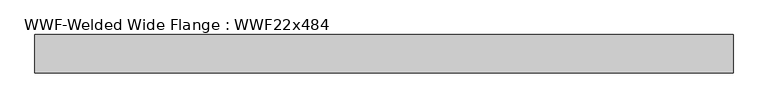
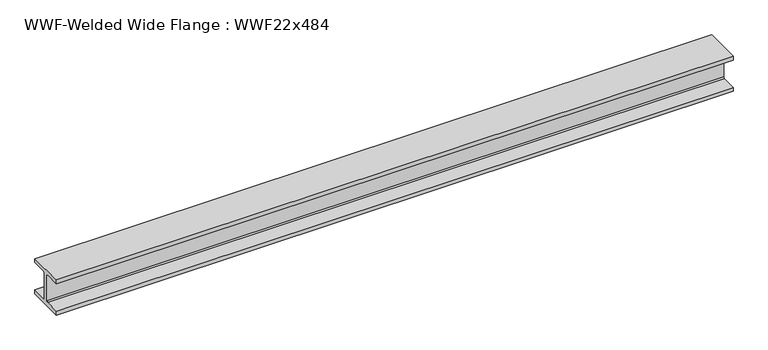
"""IFC4 building model written with IfcOpenShell, lengths in millimetres: beam geometry, WWF-Welded Wide Flange : WWF22x484."""

from ifc_helpers import new_model, si_unit, frame, origin, place, context, project, spatial, polyline, outline, extrude, source, transform, mapped, element, save


def wwf_welded_wide_flange_wwf22x484_0426b28c(model_context):
    return source(origin(), model_context, "Body", "SweptSolid", [
        extrude(outline(polyline([(274.955, -214.9602), (274.955, -274.955), (-274.955, -274.955), (-274.955, -214.9602), (-47.625, -214.9602), (-29.9974, -197.3326), (-29.9974, 197.3326), (-47.625, 214.9602), (-274.955, 214.9602), (-274.955, 274.955), (274.955, 274.955), (274.955, 214.9602), (47.625, 214.9602), (29.9974, 197.3326), (29.9974, -197.3326), (47.625, -214.9602), (274.955, -214.9602)])), frame((-5000.0, 0.0, 0.0), z_axis=(1.0, 0.0, 0.0), x_axis=(0.0, 1.0, 0.0)), (0.0, 0.0, 1.0), 10000.0),
    ])


if __name__ == "__main__":
    model = new_model("IFC4")
    model_context = context("Model", 3, world=origin())
    ifc_project = project(units=[si_unit("LENGTHUNIT", "METRE", prefix="MILLI")], contexts=[model_context])
    site = spatial("IfcSite", under=ifc_project)
    building = spatial("IfcBuilding", under=site)
    placement = place(None, origin())
    wwf_welded_wide_flange_wwf22x484_shape = wwf_welded_wide_flange_wwf22x484_0426b28c(model_context)
    element("IfcBeam", 1, ObjectType="WWF-Welded Wide Flange : WWF22x484", at=placement, inside=building, context=model_context, shape_type="MappedRepresentation", body=[
        mapped(wwf_welded_wide_flange_wwf22x484_shape, transform((0.0, 0.0, 0.0), x_axis=(1.0, 0.0, 0.0), y_axis=(0.0, 1.0, 0.0), z_axis=(0.0, 0.0, 1.0))),
    ])
    save(model, "model.ifc")

# Revit data of these elements
# Type "WWF-Welded Wide Flange : WWF22x484"
#   Assembly Code = "B10"
#   Nominal d = "12"
#   W = 484
#   Length [instance default] = 1524 mm
#   bf = 549.91 mm
#   d = 549.91 mm
#   k = 47.625 mm
#   tf = 59.995 mm
#   tw = 59.995 mm
#   A = 0.0922579 m²
#   Structural Material [instance default] = Steel ASTM A572
# Element 1 (IfcBeam, "WWF-Welded Wide Flange : WWF22x484")
#   Structural Material = Metal - Steel 43-275
#   Materials on its faces: "Metal - Steel 43-275"
# Materials
#   "Steel ASTM A572": class "Metal", colour RGB 247 247 247, transparency 0, Description = "Structural steel, high strength low alloy, ASTM - A572 - 50", Cost = 0
#   "Metal - Steel 43-275": class "Metal", colour RGB 247 247 247, transparency 0, Cost = 0
